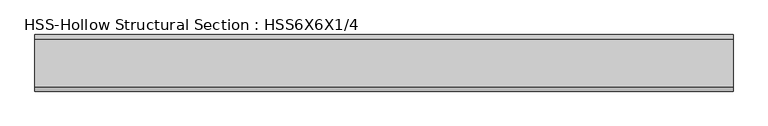
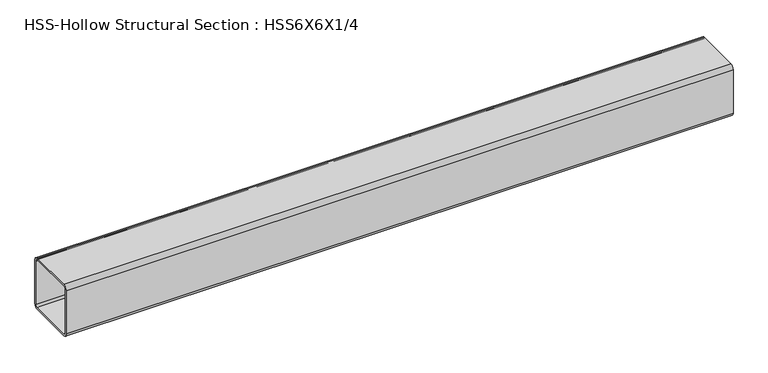
"""IFC4 building model written with IfcOpenShell, lengths in millimetres: beam geometry, HSS-Hollow Structural Section : HSS6X6X1/4."""

from ifc_helpers import new_model, si_unit, point, frame, frame_2d, origin, place, context, project, spatial, polyline, circle_curve, trimmed, segment, composite_curve, outline, extrude, source, transform, mapped, element, save


def hss_hollow_structural_section_hss6x6x1_4_49280962(model_context):
    return source(origin(), model_context, "Body", "SweptSolid", [
        extrude(outline(composite_curve([segment(polyline([(76.2, 64.3636), (76.2, -64.3636)]), True, "CONTINUOUS"), segment(trimmed(circle_curve(frame_2d((64.3636, -64.3636)), 11.8364), [point((76.2, -64.3636))], [point((64.3636, -76.2))], False, "CARTESIAN"), True, "CONTINUOUS"), segment(polyline([(64.3636, -76.2), (-64.3636, -76.2)]), True, "CONTINUOUS"), segment(trimmed(circle_curve(frame_2d((-64.3636, -64.3636)), 11.8364), [point((-64.3636, -76.2))], [point((-76.2, -64.3636))], False, "CARTESIAN"), True, "CONTINUOUS"), segment(polyline([(-76.2, -64.3636), (-76.2, 64.3636)]), True, "CONTINUOUS"), segment(trimmed(circle_curve(frame_2d((-64.3636, 64.3636)), 11.8364), [point((-76.2, 64.3636))], [point((-64.3636, 76.2))], False, "CARTESIAN"), True, "CONTINUOUS"), segment(polyline([(-64.3636, 76.2), (64.3636, 76.2)]), True, "CONTINUOUS"), segment(trimmed(circle_curve(frame_2d((64.3636, 64.3636)), 11.8364), [point((64.3636, 76.2))], [point((76.2, 64.3636))], False, "CARTESIAN"), True, "CONTINUOUS")], self_intersect=False), holes=[composite_curve([segment(trimmed(circle_curve(frame_2d((-64.3636, 64.3636)), 5.9182), [point((-64.3636, 70.2818))], [point((-70.2818, 64.3636))], True, "CARTESIAN"), True, "CONTINUOUS"), segment(polyline([(-70.2818, 64.3636), (-70.2818, -64.3636)]), True, "CONTINUOUS"), segment(trimmed(circle_curve(frame_2d((-64.3636, -64.3636)), 5.9182), [point((-70.2818, -64.3636))], [point((-64.3636, -70.2818))], True, "CARTESIAN"), True, "CONTINUOUS"), segment(polyline([(-64.3636, -70.2818), (64.3636, -70.2818)]), True, "CONTINUOUS"), segment(trimmed(circle_curve(frame_2d((64.3636, -64.3636)), 5.9182), [point((64.3636, -70.2818))], [point((70.2818, -64.3636))], True, "CARTESIAN"), True, "CONTINUOUS"), segment(polyline([(70.2818, -64.3636), (70.2818, 64.3636)]), True, "CONTINUOUS"), segment(trimmed(circle_curve(frame_2d((64.3636, 64.3636)), 5.9182), [point((70.2818, 64.3636))], [point((64.3636, 70.2818))], True, "CARTESIAN"), True, "CONTINUOUS"), segment(polyline([(64.3636, 70.2818), (-64.3636, 70.2818)]), True, "CONTINUOUS")], self_intersect=False)]), frame((-939.7939178, 0.0, 0.0), z_axis=(1.0, 0.0, 0.0), x_axis=(0.0, 1.0, 0.0)), (0.0, 0.0, 1.0), 1879.5939178),
    ])


if __name__ == "__main__":
    model = new_model("IFC4")
    model_context = context("Model", 3, world=origin())
    ifc_project = project(units=[si_unit("LENGTHUNIT", "METRE", prefix="MILLI")], contexts=[model_context])
    site = spatial("IfcSite", under=ifc_project)
    building = spatial("IfcBuilding", under=site)
    placement = place(None, origin())
    hss_hollow_structural_section_hss6x6x1_4_shape = hss_hollow_structural_section_hss6x6x1_4_49280962(model_context)
    element("IfcBeam", 1, ObjectType="HSS-Hollow Structural Section : HSS6X6X1/4", at=placement, inside=building, context=model_context, shape_type="MappedRepresentation", body=[
        mapped(hss_hollow_structural_section_hss6x6x1_4_shape, transform((0.0, 0.0, 0.0), x_axis=(1.0, 0.0, 0.0), y_axis=(0.0, 1.0, 0.0), z_axis=(0.0, 0.0, 1.0))),
    ])
    save(model, "model.ifc")

# Revit data of these elements
# Type "HSS-Hollow Structural Section : HSS6X6X1/4"
#   Assembly Code = "B10"
#   Shape = "Square"
#   W = 19
#   Ht = 0' - 6"
#   Length [instance default] = 5' - 0"
#   b = 0' - 6"
#   kr = 0' - 0.466"
#   t = 0' - 0.233"
#   A = 0.0363889 SF
#   Structural Material [instance default] = Steel ASTM A500, Grade B, Rectangular and Square
# Element 1 (IfcBeam, "HSS-Hollow Structural Section : HSS6X6X1/4")
#   Materials on its faces: "Steel ASTM A500, Grade B, Rectangular and Square"
# Materials
#   "Steel ASTM A500, Grade B, Rectangular and Square": class "Metal", colour RGB 199 199 199, transparency 0, Description = "Carbon steel", Cost = 0
